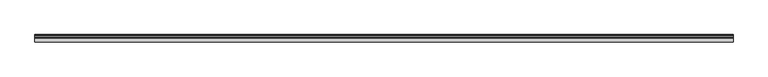
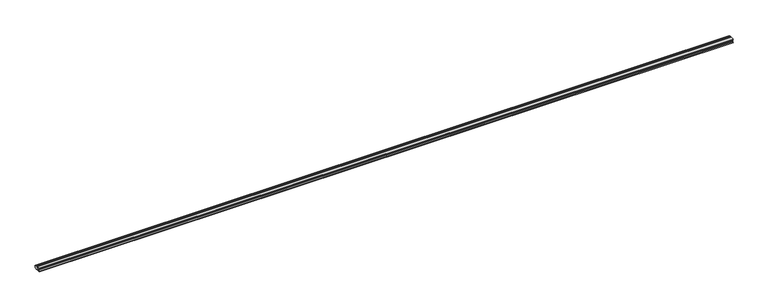
"""IFC4 building model written with IfcOpenShell, lengths in millimetres: proxy geometry, Generic Models 6:Generic Models 2:318829:Generic Models 2:318829 : Generic Models 6:Generic Models 2:318829:7 : Generic Models 6:Generic Models 2:318829:Generic Models 2:318829 : Generic Models 6:Generic Models 2:318829:300683."""

from ifc_helpers import new_model, si_unit, frame, origin, place, context, project, spatial, polyline, outline, extrude, source, transform, mapped, element, save


def generic_models_fd9d2638(model_context):
    return source(origin(), model_context, "Body", "SweptSolid", [
        extrude(outline(polyline([(-579074.6633115, 3698.9870698), (-579086.3994958, 3698.9870698), (-579085.6446786, 3700.9185962), (-579085.0173064, 3705.3370698), (-579085.6446786, 3709.7555433), (-579086.3994958, 3711.6870698), (-579074.6633115, 3711.6870698), (-579077.849745, 3709.9214921), (-579079.7981551, 3707.4387239), (-579080.2037308, 3704.6271713), (-579079.0030238, 3701.9266758), (-579076.3838735, 3699.7597049), (-579074.6633115, 3698.9870698)])), frame((590317.0242239, 0.0, 0.0), z_axis=(1.0, 0.0, 0.0), x_axis=(0.0, 1.0, 0.0)), (0.0, 0.0, 1.0), 2438.4),
        extrude(outline(polyline([(-579067.8165445, 3699.1462775), (-579069.9360564, 3698.9870698), (-579072.0555683, 3699.1462775), (-579075.8747968, 3700.3724399), (-579078.5177849, 3702.581908), (-579079.4610564, 3705.3370698), (-579078.5177849, 3708.0922315), (-579075.8747968, 3710.3016997), (-579072.0555683, 3711.527862), (-579069.9360564, 3711.6870698), (-579067.8165445, 3711.527862), (-579063.997316, 3710.3016997), (-579061.3543279, 3708.0922315), (-579060.4110564, 3705.3370698), (-579061.3543279, 3702.581908), (-579063.997316, 3700.3724399), (-579067.8165445, 3699.1462775)])), frame((590317.0242239, 0.0, 0.0), z_axis=(1.0, 0.0, 0.0), x_axis=(0.0, 1.0, 0.0)), (0.0, 0.0, 1.0), 2438.4),
    ])


if __name__ == "__main__":
    model = new_model("IFC4")
    model_context = context("Model", 3, world=origin())
    ifc_project = project(units=[si_unit("LENGTHUNIT", "METRE", prefix="MILLI")], contexts=[model_context])
    site = spatial("IfcSite", under=ifc_project)
    building = spatial("IfcBuilding", under=site)
    placement = place(None, origin())
    generic_models_shape = generic_models_fd9d2638(model_context)
    element("IfcBuildingElementProxy", 1, Name="Generic Models 6:Generic Models 2:318829:Generic Models 2:318829 : Generic Models 6:Generic Models 2:318829:7 : Generic Models 6:Generic Models 2:318829:Generic Models 2:318829 : Generic Models 6:Generic Models 2:318829:300683", ObjectType="Generic Models 6:Generic Models 2:318829:Generic Models 2:318829 : Generic Models 6:Generic Models 2:318829:7 : Generic Models 6:Generic Models 2:318829:Generic Models 2:318829 : Generic Models 6:Generic Models 2:318829:300683", at=placement, inside=building, context=model_context, shape_type="MappedRepresentation", body=[
        mapped(generic_models_shape, transform((0.0, 0.0, 0.0), x_axis=(1.0, 0.0, 0.0), y_axis=(0.0, 1.0, 0.0), z_axis=(0.0, 0.0, 1.0))),
    ])
    save(model, "model.ifc")

# Revit data of these elements
# Type "Generic Models 6:Generic Models 2:318829:Generic Models 2:318829 : Generic Models 6:Generic Models 2:318829:7 : Generic Models 6:Generic Models 2:318829:Generic Models 2:318829 : Generic Models 6:Generic Models 2:318829:300683"
#   NameOverride = "Generic Models 6:Generic Models 2:318829:Generic Models 2:318829 : Generic Models 6:Generic Models 2:318829:300683"
#   ObjectTypeOverride = "Generic Models 2:318829 : Generic Models 6:Generic Models 2:318829"
#   Reference = "Generic Models 2"
#   Tag = "300683"
# Element 1 (IfcBuildingElementProxy, "Generic Models 6:Generic Models 2:318829:Generic Models 2:318829 : Generic Models 6:Generic Models 2:318829:7 : Generic Models 6:Generic Models 2:318829:Generic Models 2:318829 : Generic Models 6:Generic Models 2:318829:300683")
#   Materials on its faces: "SEALANT & BACKER ROD, IF NECESSARY"
# Materials
#   "SEALANT & BACKER ROD, IF NECESSARY": class "Unassigned", colour RGB 120 120 120, transparency 0, Cost = 0
